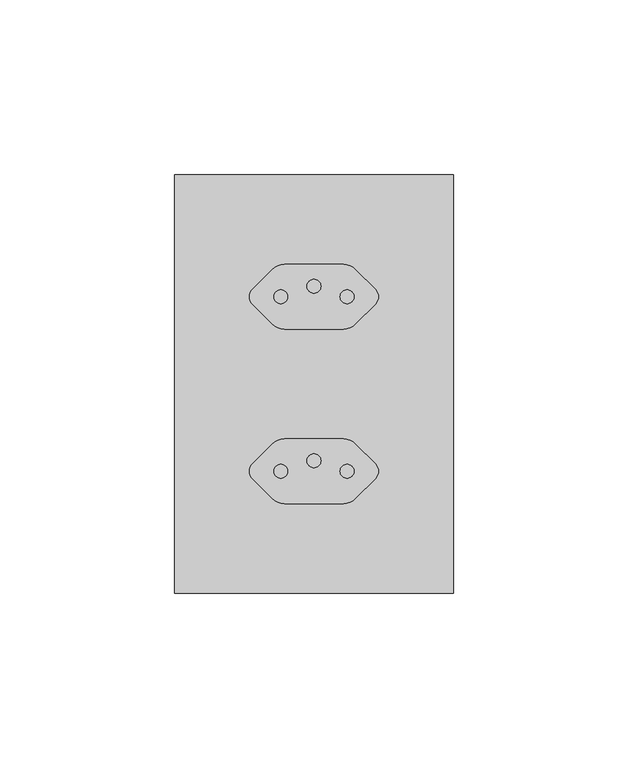
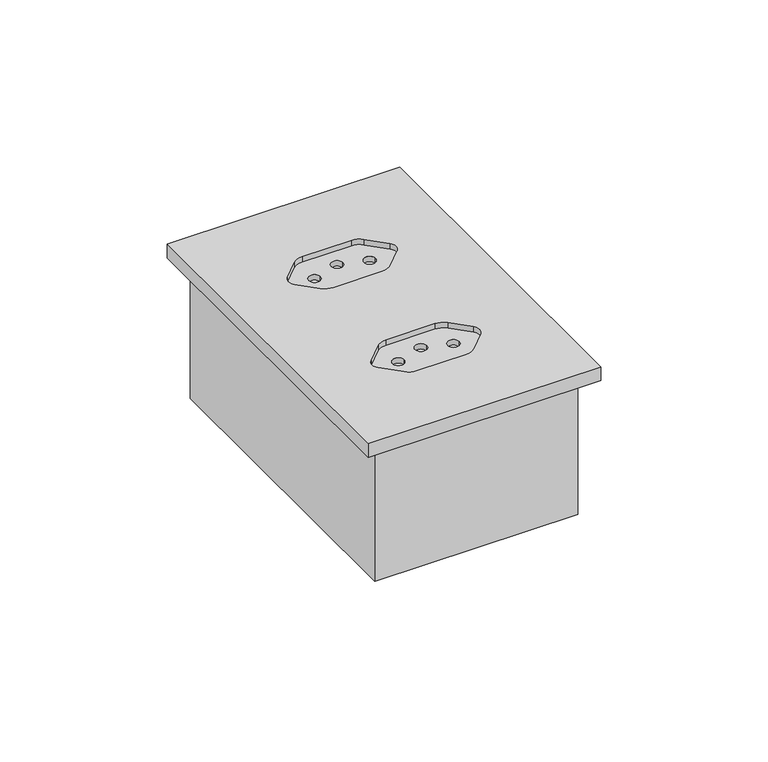
"""IFC4 building model written with IfcOpenShell, lengths in millimetres: proxy geometry, CAIXA VERTICE V7 : Tomada 10A 2s."""

from ifc_helpers import new_model, si_unit, frame, origin, place, context, project, spatial, polyline, circle_curve, faceted_brep, source, transform, mapped, element, save
from ifc_brep_helpers import plane_surface, revolved_surface, advanced_brep


def electrical_fixtures_e68da447(model_context):
    return source(origin(), model_context, "Body", "SolidModel", [
        faceted_brep([(33.0, 1047.0, -48.0), (33.0, 1153.0, -48.0), (-33.0, 1153.0, -48.0), (-33.0, 1047.0, -48.0), (35.0, 1155.0, -50.0), (35.0, 1045.0, -50.0), (-35.0, 1045.0, -50.0), (-35.0, 1155.0, -50.0), (-35.0, 1155.0, 0.0), (35.0, 1155.0, 0.0), (-35.0, 1045.0, 0.0), (35.0, 1045.0, 0.0), (33.0, 1153.0, 0.0), (33.0, 1047.0, 0.0), (-33.0, 1047.0, 0.0), (-33.0, 1153.0, 0.0)], [[[0, 1, 2, 3]], [[4, 5, 6, 7]], [[4, 7, 8, 9]], [[8, 7, 6, 10]], [[10, 6, 5, 11]], [[11, 5, 4, 9]], [[9, 8, 10, 11], [12, 13, 14, 15]], [[13, 12, 1, 0]], [[14, 13, 0, 3]], [[15, 14, 3, 2]], [[12, 15, 2, 1]]]),
        advanced_brep(
        [(40.0, 1160.0, 5.0), (-40.0, 1160.0, 5.0), (-40.0, 1040.0, 5.0), (40.0, 1040.0, 5.0), (8.4215729, 1115.75, 5.0), (-8.4215729, 1115.75, 5.0), (-11.9571068, 1117.2144661, 5.0), (-17.6213203, 1122.8786797, 5.0), (-17.6213203, 1127.1213203, 5.0), (-11.9571068, 1132.7855339, 5.0), (-8.4215729, 1134.25, 5.0), (8.4215729, 1134.25, 5.0), (11.9571068, 1132.7855339, 5.0), (17.6213203, 1127.1213203, 5.0), (17.6213203, 1122.8786797, 5.0), (11.9571068, 1117.2144661, 5.0), (8.4215729, 1065.75, 5.0), (-8.4215729, 1065.75, 5.0), (-11.9571068, 1067.2144661, 5.0), (-17.6213203, 1072.8786797, 5.0), (-17.6213203, 1077.1213203, 5.0), (-11.9571068, 1082.7855339, 5.0), (-8.4215729, 1084.25, 5.0), (8.4215729, 1084.25, 5.0), (11.9571068, 1082.7855339, 5.0), (17.6213203, 1077.1213203, 5.0), (17.6213203, 1072.8786797, 5.0), (11.9571068, 1067.2144661, 5.0), (-40.0, 1160.0, 0.0), (40.0, 1160.0, 0.0), (40.0, 1040.0, 0.0), (-40.0, 1040.0, 0.0), (8.4215729, 1115.75, 3.0), (11.9571068, 1117.2144661, 3.0), (17.6213203, 1122.8786797, 3.0), (17.6213203, 1127.1213203, 3.0), (11.9571068, 1132.7855339, 3.0), (8.4215729, 1134.25, 3.0), (-8.4215729, 1134.25, 3.0), (-11.9571068, 1132.7855339, 3.0), (-17.6213203, 1127.1213203, 3.0), (-17.6213203, 1122.8786797, 3.0), (-11.9571068, 1117.2144661, 3.0), (-8.4215729, 1115.75, 3.0), (-7.5, 1125.0, 3.0), (-11.5, 1125.0, 3.0), (11.5, 1125.0, 3.0), (7.5, 1125.0, 3.0), (2.0, 1128.0, 3.0), (-2.0, 1128.0, 3.0), (-11.5, 1125.0, 1.0), (-7.5, 1125.0, 1.0), (7.5, 1125.0, 1.0), (11.5, 1125.0, 1.0), (-2.0, 1128.0, 1.0), (2.0, 1128.0, 1.0), (8.4215729, 1065.75, 3.0), (11.9571068, 1067.2144661, 3.0), (17.6213203, 1072.8786797, 3.0), (17.6213203, 1077.1213203, 3.0), (11.9571068, 1082.7855339, 3.0), (8.4215729, 1084.25, 3.0), (-8.4215729, 1084.25, 3.0), (-11.9571068, 1082.7855339, 3.0), (-17.6213203, 1077.1213203, 3.0), (-17.6213203, 1072.8786797, 3.0), (-11.9571068, 1067.2144661, 3.0), (-8.4215729, 1065.75, 3.0), (-7.5, 1075.0, 3.0), (-11.5, 1075.0, 3.0), (11.5, 1075.0, 3.0), (7.5, 1075.0, 3.0), (2.0, 1078.0, 3.0), (-2.0, 1078.0, 3.0), (-11.5, 1075.0, 1.0), (-7.5, 1075.0, 1.0), (7.5, 1075.0, 1.0), (11.5, 1075.0, 1.0), (-2.0, 1078.0, 1.0), (2.0, 1078.0, 1.0)],
        [
            (0, 1),
            (1, 2),
            (2, 3),
            (3, 0),
            (4, 5),
            (5, 6, circle_curve(frame((-8.4215729, 1120.75, 5.0), z_axis=(0.0, 0.0, -1.0), x_axis=(-1.0, 0.0, 0.0)), 5.0)),
            (6, 7),
            (7, 8, circle_curve(frame((-15.5, 1125.0, 5.0), z_axis=(0.0, 0.0, -1.0), x_axis=(-1.0, 0.0, 0.0)), 3.0)),
            (8, 9),
            (9, 10, circle_curve(frame((-8.4215729, 1129.25, 5.0), z_axis=(0.0, 0.0, -1.0), x_axis=(-1.0, 0.0, 0.0)), 5.0)),
            (10, 11),
            (11, 12, circle_curve(frame((8.4215729, 1129.25, 5.0), z_axis=(0.0, 0.0, -1.0), x_axis=(-1.0, 0.0, 0.0)), 5.0)),
            (12, 13),
            (13, 14, circle_curve(frame((15.5, 1125.0, 5.0), z_axis=(0.0, 0.0, -1.0), x_axis=(-1.0, 0.0, 0.0)), 3.0)),
            (14, 15),
            (15, 4, circle_curve(frame((8.4215729, 1120.75, 5.0), z_axis=(0.0, 0.0, -1.0), x_axis=(-1.0, 0.0, 0.0)), 5.0)),
            (16, 17),
            (17, 18, circle_curve(frame((-8.4215729, 1070.75, 5.0), z_axis=(0.0, 0.0, -1.0), x_axis=(-1.0, 0.0, 0.0)), 5.0)),
            (18, 19),
            (19, 20, circle_curve(frame((-15.5, 1075.0, 5.0), z_axis=(0.0, 0.0, -1.0), x_axis=(-1.0, 0.0, 0.0)), 3.0)),
            (20, 21),
            (21, 22, circle_curve(frame((-8.4215729, 1079.25, 5.0), z_axis=(0.0, 0.0, -1.0), x_axis=(-1.0, 0.0, 0.0)), 5.0)),
            (22, 23),
            (23, 24, circle_curve(frame((8.4215729, 1079.25, 5.0), z_axis=(0.0, 0.0, -1.0), x_axis=(-1.0, 0.0, 0.0)), 5.0)),
            (24, 25),
            (25, 26, circle_curve(frame((15.5, 1075.0, 5.0), z_axis=(0.0, 0.0, -1.0), x_axis=(-1.0, 0.0, 0.0)), 3.0)),
            (26, 27),
            (27, 16, circle_curve(frame((8.4215729, 1070.75, 5.0), z_axis=(0.0, 0.0, -1.0), x_axis=(-1.0, 0.0, 0.0)), 5.0)),
            (28, 29),
            (29, 30),
            (30, 31),
            (31, 28),
            (0, 29),
            (28, 1),
            (31, 2),
            (30, 3),
            (32, 33, circle_curve(frame((8.4215729, 1120.75, 3.0), z_axis=(0.0, 0.0, 1.0), x_axis=(-1.0, 0.0, 0.0)), 5.0)),
            (33, 34),
            (34, 35, circle_curve(frame((15.5, 1125.0, 3.0), z_axis=(0.0, 0.0, 1.0), x_axis=(-1.0, 0.0, 0.0)), 3.0)),
            (35, 36),
            (36, 37, circle_curve(frame((8.4215729, 1129.25, 3.0), z_axis=(0.0, 0.0, 1.0), x_axis=(-1.0, 0.0, 0.0)), 5.0)),
            (37, 38),
            (38, 39, circle_curve(frame((-8.4215729, 1129.25, 3.0), z_axis=(0.0, 0.0, 1.0), x_axis=(-1.0, 0.0, 0.0)), 5.0)),
            (39, 40),
            (40, 41, circle_curve(frame((-15.5, 1125.0, 3.0), z_axis=(0.0, 0.0, 1.0), x_axis=(-1.0, 0.0, 0.0)), 3.0)),
            (41, 42),
            (42, 43, circle_curve(frame((-8.4215729, 1120.75, 3.0), z_axis=(0.0, 0.0, 1.0), x_axis=(-1.0, 0.0, 0.0)), 5.0)),
            (43, 32),
            (44, 45, circle_curve(frame((-9.5, 1125.0, 3.0), z_axis=(0.0, 0.0, -1.0), x_axis=(1.0, 2.301812013077709e-12, 0.0)), 2.0)),
            (45, 44, circle_curve(frame((-9.5, 1125.0, 3.0), z_axis=(0.0, 0.0, -1.0), x_axis=(1.0, 2.301812013077709e-12, 0.0)), 2.0)),
            (46, 47, circle_curve(frame((9.5, 1125.0, 3.0), z_axis=(0.0, 0.0, -1.0), x_axis=(1.0, 2.301812013077709e-12, 0.0)), 2.0)),
            (47, 46, circle_curve(frame((9.5, 1125.0, 3.0), z_axis=(0.0, 0.0, -1.0), x_axis=(1.0, 2.301812013077709e-12, 0.0)), 2.0)),
            (48, 49, circle_curve(frame((0.0, 1128.0, 3.0), z_axis=(0.0, 0.0, -1.0), x_axis=(1.0, 2.301812013077709e-12, 0.0)), 2.0)),
            (49, 48, circle_curve(frame((0.0, 1128.0, 3.0), z_axis=(0.0, 0.0, -1.0), x_axis=(1.0, 2.301812013077709e-12, 0.0)), 2.0)),
            (43, 5),
            (4, 32),
            (42, 6),
            (41, 7),
            (40, 8),
            (39, 9),
            (38, 10),
            (37, 11),
            (36, 12),
            (35, 13),
            (34, 14),
            (33, 15),
            (50, 51, circle_curve(frame((-9.5, 1125.0, 1.0), z_axis=(0.0, 0.0, 1.0), x_axis=(1.0, 2.301812013077709e-12, 0.0)), 2.0)),
            (51, 50, circle_curve(frame((-9.5, 1125.0, 1.0), z_axis=(0.0, 0.0, 1.0), x_axis=(1.0, 2.301812013077709e-12, 0.0)), 2.0)),
            (52, 53, circle_curve(frame((9.5, 1125.0, 1.0), z_axis=(0.0, 0.0, 1.0), x_axis=(1.0, 2.301812013077709e-12, 0.0)), 2.0)),
            (53, 52, circle_curve(frame((9.5, 1125.0, 1.0), z_axis=(0.0, 0.0, 1.0), x_axis=(1.0, 2.301812013077709e-12, 0.0)), 2.0)),
            (54, 55, circle_curve(frame((0.0, 1128.0, 1.0), z_axis=(0.0, 0.0, 1.0), x_axis=(1.0, 2.301812013077709e-12, 0.0)), 2.0)),
            (55, 54, circle_curve(frame((0.0, 1128.0, 1.0), z_axis=(0.0, 0.0, 1.0), x_axis=(1.0, 2.301812013077709e-12, 0.0)), 2.0)),
            (44, 51),
            (50, 45),
            (46, 53),
            (52, 47),
            (48, 55),
            (54, 49),
            (56, 57, circle_curve(frame((8.4215729, 1070.75, 3.0), z_axis=(0.0, 0.0, 1.0), x_axis=(-1.0, 0.0, 0.0)), 5.0)),
            (57, 58),
            (58, 59, circle_curve(frame((15.5, 1075.0, 3.0), z_axis=(0.0, 0.0, 1.0), x_axis=(-1.0, 0.0, 0.0)), 3.0)),
            (59, 60),
            (60, 61, circle_curve(frame((8.4215729, 1079.25, 3.0), z_axis=(0.0, 0.0, 1.0), x_axis=(-1.0, 0.0, 0.0)), 5.0)),
            (61, 62),
            (62, 63, circle_curve(frame((-8.4215729, 1079.25, 3.0), z_axis=(0.0, 0.0, 1.0), x_axis=(-1.0, 0.0, 0.0)), 5.0)),
            (63, 64),
            (64, 65, circle_curve(frame((-15.5, 1075.0, 3.0), z_axis=(0.0, 0.0, 1.0), x_axis=(-1.0, 0.0, 0.0)), 3.0)),
            (65, 66),
            (66, 67, circle_curve(frame((-8.4215729, 1070.75, 3.0), z_axis=(0.0, 0.0, 1.0), x_axis=(-1.0, 0.0, 0.0)), 5.0)),
            (67, 56),
            (68, 69, circle_curve(frame((-9.5, 1075.0, 3.0), z_axis=(0.0, 0.0, -1.0), x_axis=(1.0, 2.301812013077709e-12, 0.0)), 2.0)),
            (69, 68, circle_curve(frame((-9.5, 1075.0, 3.0), z_axis=(0.0, 0.0, -1.0), x_axis=(1.0, 2.301812013077709e-12, 0.0)), 2.0)),
            (70, 71, circle_curve(frame((9.5, 1075.0, 3.0), z_axis=(0.0, 0.0, -1.0), x_axis=(1.0, 2.301812013077709e-12, 0.0)), 2.0)),
            (71, 70, circle_curve(frame((9.5, 1075.0, 3.0), z_axis=(0.0, 0.0, -1.0), x_axis=(1.0, 2.301812013077709e-12, 0.0)), 2.0)),
            (72, 73, circle_curve(frame((0.0, 1078.0, 3.0), z_axis=(0.0, 0.0, -1.0), x_axis=(1.0, 2.301812013077709e-12, 0.0)), 2.0)),
            (73, 72, circle_curve(frame((0.0, 1078.0, 3.0), z_axis=(0.0, 0.0, -1.0), x_axis=(1.0, 2.301812013077709e-12, 0.0)), 2.0)),
            (67, 17),
            (16, 56),
            (66, 18),
            (65, 19),
            (64, 20),
            (63, 21),
            (62, 22),
            (61, 23),
            (60, 24),
            (59, 25),
            (58, 26),
            (57, 27),
            (74, 75, circle_curve(frame((-9.5, 1075.0, 1.0), z_axis=(0.0, 0.0, 1.0), x_axis=(1.0, 2.301812013077709e-12, 0.0)), 2.0)),
            (75, 74, circle_curve(frame((-9.5, 1075.0, 1.0), z_axis=(0.0, 0.0, 1.0), x_axis=(1.0, 2.301812013077709e-12, 0.0)), 2.0)),
            (76, 77, circle_curve(frame((9.5, 1075.0, 1.0), z_axis=(0.0, 0.0, 1.0), x_axis=(1.0, 2.301812013077709e-12, 0.0)), 2.0)),
            (77, 76, circle_curve(frame((9.5, 1075.0, 1.0), z_axis=(0.0, 0.0, 1.0), x_axis=(1.0, 2.301812013077709e-12, 0.0)), 2.0)),
            (78, 79, circle_curve(frame((0.0, 1078.0, 1.0), z_axis=(0.0, 0.0, 1.0), x_axis=(1.0, 2.301812013077709e-12, 0.0)), 2.0)),
            (79, 78, circle_curve(frame((0.0, 1078.0, 1.0), z_axis=(0.0, 0.0, 1.0), x_axis=(1.0, 2.301812013077709e-12, 0.0)), 2.0)),
            (68, 75),
            (74, 69),
            (70, 77),
            (76, 71),
            (72, 79),
            (78, 73),
        ],
        [
            plane_surface(frame((-60.0, 1160.0, 5.0), z_axis=(0.0, 0.0, 1.0), x_axis=(-1.0, 0.0, 0.0))),
            plane_surface(frame((-60.0, 1160.0, 0.0), z_axis=(0.0, 0.0, -1.0), x_axis=(1.0, 0.0, 0.0))),
            plane_surface(frame((40.0, 1160.0, 5.0), z_axis=(0.0, 1.0, 0.0), x_axis=(0.0, 0.0, -1.0))),
            plane_surface(frame((-40.0, 1160.0, 5.0), z_axis=(-1.0, 0.0, 0.0), x_axis=(0.0, 0.0, -1.0))),
            plane_surface(frame((-40.0, 1040.0, 5.0), z_axis=(0.0, -1.0, 0.0), x_axis=(0.0, 0.0, -1.0))),
            plane_surface(frame((40.0, 1040.0, 5.0), z_axis=(1.0, 0.0, 0.0), x_axis=(0.0, 0.0, -1.0))),
            plane_surface(frame((3.4215729, 1120.75, 3.0), z_axis=(0.0, 0.0, 1.0), x_axis=(0.0, 1.0, 0.0))),
            plane_surface(frame((-8.4215729, 1115.75, 5.0), z_axis=(0.0, 1.0, 0.0), x_axis=(0.0, 0.0, -1.0))),
            revolved_surface(polyline([(-13.4215729, 1120.75, 5.0), (-13.4215729, 1120.75, 3.0)]), (-8.4215729, 1120.75, 3.0), (0.0, 0.0, 1.0)),
            plane_surface(frame((-17.6213203, 1122.8786797, 5.0), z_axis=(0.7071067811865045, 0.7071067811865905, 0.0), x_axis=(0.0, 0.0, -1.0))),
            revolved_surface(polyline([(-18.5, 1125.0, 5.0), (-18.5, 1125.0, 3.0)]), (-15.5, 1125.0, 3.0), (0.0, 0.0, 1.0)),
            plane_surface(frame((-11.9571068, 1132.7855339, 5.0), z_axis=(0.7071067811865515, -0.7071067811865437, 0.0), x_axis=(0.0, 0.0, -1.0))),
            revolved_surface(polyline([(-13.4215729, 1129.25, 5.0), (-13.4215729, 1129.25, 3.0)]), (-8.4215729, 1129.25, 3.0), (0.0, 0.0, 1.0)),
            plane_surface(frame((8.4215729, 1134.25, 5.0), z_axis=(0.0, -1.0, 0.0), x_axis=(0.0, 0.0, -1.0))),
            revolved_surface(polyline([(3.4215728999999993, 1129.25, 5.0), (3.4215728999999993, 1129.25, 3.0)]), (8.4215729, 1129.25, 3.0), (0.0, 0.0, 1.0)),
            plane_surface(frame((17.6213203, 1127.1213203, 5.0), z_axis=(-0.7071067811865307, -0.7071067811865643, 0.0), x_axis=(0.0, 0.0, -1.0))),
            revolved_surface(polyline([(12.5, 1125.0, 5.0), (12.5, 1125.0, 3.0)]), (15.5, 1125.0, 3.0), (0.0, 0.0, 1.0)),
            plane_surface(frame((11.9571068, 1117.2144661, 5.0), z_axis=(-0.7071067811865893, 0.7071067811865058, 0.0), x_axis=(0.0, 0.0, -1.0))),
            revolved_surface(polyline([(3.4215728999999993, 1120.75, 5.0), (3.4215728999999993, 1120.75, 3.0)]), (8.4215729, 1120.75, 3.0), (0.0, 0.0, 1.0)),
            plane_surface(frame((-7.5, 1125.0, 1.0), z_axis=(0.0, 0.0, 1.0), x_axis=(2.301812013077709e-12, -1.0, 0.0))),
            revolved_surface(polyline([(-7.5, 1125.0000000000045, 3.0), (-7.5, 1125.0000000000045, 1.0)]), (-9.5, 1125.0, 1.0), (0.0, 0.0, 1.0)),
            revolved_surface(polyline([(11.5, 1125.0000000000045, 3.0), (11.5, 1125.0000000000045, 1.0)]), (9.5, 1125.0, 5.0), (0.0, 0.0, 1.0)),
            revolved_surface(polyline([(2.0, 1128.0000000000045, 3.0), (2.0, 1128.0000000000045, 1.0)]), (0.0, 1128.0, 5.0), (0.0, 0.0, 1.0)),
            plane_surface(frame((3.4215729, 1070.75, 3.0), z_axis=(0.0, 0.0, 1.0), x_axis=(0.0, 1.0, 0.0))),
            plane_surface(frame((-8.4215729, 1065.75, 5.0), z_axis=(0.0, 1.0, 0.0), x_axis=(0.0, 0.0, -1.0))),
            revolved_surface(polyline([(-13.4215729, 1070.75, 5.0), (-13.4215729, 1070.75, 3.0)]), (-8.4215729, 1070.75, 3.0), (0.0, 0.0, 1.0)),
            plane_surface(frame((-17.6213203, 1072.8786797, 5.0), z_axis=(0.7071067811865045, 0.7071067811865905, 0.0), x_axis=(0.0, 0.0, -1.0))),
            revolved_surface(polyline([(-18.5, 1075.0, 5.0), (-18.5, 1075.0, 3.0)]), (-15.5, 1075.0, 3.0), (0.0, 0.0, 1.0)),
            plane_surface(frame((-11.9571068, 1082.7855339, 5.0), z_axis=(0.7071067811865515, -0.7071067811865437, 0.0), x_axis=(0.0, 0.0, -1.0))),
            revolved_surface(polyline([(-13.4215729, 1079.25, 5.0), (-13.4215729, 1079.25, 3.0)]), (-8.4215729, 1079.25, 3.0), (0.0, 0.0, 1.0)),
            plane_surface(frame((8.4215729, 1084.25, 5.0), z_axis=(0.0, -1.0, 0.0), x_axis=(0.0, 0.0, -1.0))),
            revolved_surface(polyline([(3.4215728999999993, 1079.25, 5.0), (3.4215728999999993, 1079.25, 3.0)]), (8.4215729, 1079.25, 3.0), (0.0, 0.0, 1.0)),
            plane_surface(frame((17.6213203, 1077.1213203, 5.0), z_axis=(-0.7071067811865307, -0.7071067811865643, 0.0), x_axis=(0.0, 0.0, -1.0))),
            revolved_surface(polyline([(12.5, 1075.0, 5.0), (12.5, 1075.0, 3.0)]), (15.5, 1075.0, 3.0), (0.0, 0.0, 1.0)),
            plane_surface(frame((11.9571068, 1067.2144661, 5.0), z_axis=(-0.7071067811865893, 0.7071067811865058, 0.0), x_axis=(0.0, 0.0, -1.0))),
            revolved_surface(polyline([(3.4215728999999993, 1070.75, 5.0), (3.4215728999999993, 1070.75, 3.0)]), (8.4215729, 1070.75, 3.0), (0.0, 0.0, 1.0)),
            plane_surface(frame((-7.5, 1075.0, 1.0), z_axis=(0.0, 0.0, 1.0), x_axis=(2.301812013077709e-12, -1.0, 0.0))),
            revolved_surface(polyline([(-7.5, 1075.0000000000045, 3.0), (-7.5, 1075.0000000000045, 1.0)]), (-9.5, 1075.0, 1.0), (0.0, 0.0, 1.0)),
            revolved_surface(polyline([(11.5, 1075.0000000000045, 3.0), (11.5, 1075.0000000000045, 1.0)]), (9.5, 1075.0, 5.0), (0.0, 0.0, 1.0)),
            revolved_surface(polyline([(2.0, 1078.0000000000045, 3.0), (2.0, 1078.0000000000045, 1.0)]), (0.0, 1078.0, 5.0), (0.0, 0.0, 1.0)),
        ],
        [
            (0, [[1, 2, 3, 4], [5, 6, 7, 8, 9, 10, 11, 12, 13, 14, 15, 16], [17, 18, 19, 20, 21, 22, 23, 24, 25, 26, 27, 28]]),
            (1, [[29, 30, 31, 32]]),
            (2, [[-1, 33, -29, 34]]),
            (3, [[-2, -34, -32, 35]]),
            (4, [[-3, -35, -31, 36]]),
            (5, [[-4, -36, -30, -33]]),
            (6, [[37, 38, 39, 40, 41, 42, 43, 44, 45, 46, 47, 48], [49, 50], [51, 52], [53, 54]]),
            (7, [[-48, 55, -5, 56]]),
            (8, [[-47, 57, -6, -55]]),
            (9, [[-46, 58, -7, -57]]),
            (10, [[-45, 59, -8, -58]]),
            (11, [[-44, 60, -9, -59]]),
            (12, [[-43, 61, -10, -60]]),
            (13, [[-42, 62, -11, -61]]),
            (14, [[-41, 63, -12, -62]]),
            (15, [[-40, 64, -13, -63]]),
            (16, [[-39, 65, -14, -64]]),
            (17, [[-38, 66, -15, -65]]),
            (18, [[-37, -56, -16, -66]]),
            (19, [[67, 68]]),
            (19, [[69, 70]]),
            (19, [[71, 72]]),
            (20, [[-49, 73, -67, 74]]),
            (20, [[-50, -74, -68, -73]]),
            (21, [[-51, 75, -69, 76]]),
            (21, [[-52, -76, -70, -75]]),
            (22, [[-53, 77, -71, 78]]),
            (22, [[-54, -78, -72, -77]]),
            (23, [[79, 80, 81, 82, 83, 84, 85, 86, 87, 88, 89, 90], [91, 92], [93, 94], [95, 96]]),
            (24, [[-90, 97, -17, 98]]),
            (25, [[-89, 99, -18, -97]]),
            (26, [[-88, 100, -19, -99]]),
            (27, [[-87, 101, -20, -100]]),
            (28, [[-86, 102, -21, -101]]),
            (29, [[-85, 103, -22, -102]]),
            (30, [[-84, 104, -23, -103]]),
            (31, [[-83, 105, -24, -104]]),
            (32, [[-82, 106, -25, -105]]),
            (33, [[-81, 107, -26, -106]]),
            (34, [[-80, 108, -27, -107]]),
            (35, [[-79, -98, -28, -108]]),
            (36, [[109, 110]]),
            (36, [[111, 112]]),
            (36, [[113, 114]]),
            (37, [[-91, 115, -109, 116]]),
            (37, [[-92, -116, -110, -115]]),
            (38, [[-93, 117, -111, 118]]),
            (38, [[-94, -118, -112, -117]]),
            (39, [[-95, 119, -113, 120]]),
            (39, [[-96, -120, -114, -119]]),
        ],
    ),
    ])


if __name__ == "__main__":
    model = new_model("IFC4")
    model_context = context("Model", 3, world=origin())
    ifc_project = project(units=[si_unit("LENGTHUNIT", "METRE", prefix="MILLI")], contexts=[model_context])
    site = spatial("IfcSite", under=ifc_project)
    building = spatial("IfcBuilding", under=site)
    placement = place(None, origin())
    electrical_fixtures_shape = electrical_fixtures_e68da447(model_context)
    element("IfcBuildingElementProxy", 1, Name="CAIXA VERTICE V7 : Tomada 10A 2s", ObjectType="CAIXA VERTICE V7 : Tomada 10A 2s", at=placement, inside=building, context=model_context, shape_type="MappedRepresentation", body=[
        mapped(electrical_fixtures_shape, transform((0.0, 0.0, 0.0), x_axis=(1.0, 0.0, 0.0), y_axis=(0.0, 1.0, 0.0), z_axis=(0.0, 0.0, 1.0))),
    ])
    save(model, "model.ifc")

# Revit data of these elements
# Type "CAIXA VERTICE V7 : Tomada 10A 2s"
#   URL = "www.facebook.com/verticetreinamentos"
#   SEÇÃO [instance default] = ""
#   Rotação [instance default] = 0.00°
#   LARGURA DA TAMPA = 0.08 m
#   BORDA = 0.01 m
#   ALTURA DE INSTALAÇÃO [instance default] = 1.10 m
#   Distância Anotação [instance default] = 0.0015 m
#   ALTURA DA TAMPA = 0.12 m
#   Vertical [instance default] = yes
#   VER SEÇÃO [instance default] = no
#   SHADE ESQ [instance default] = no
#   SHADE DIR [instance default] = yes
#   HORIZONTAL [instance default] = no
#   ANDAR COM A LEGENDA [instance default] = 0
#   Material Tampa [instance default] = Plástico, branco opaco
#   Caixa = element 1798515
#   Anotação = element 1798529
#   Default Elevation = 0
# Element 1 (IfcBuildingElementProxy, "CAIXA VERTICE V7 : Tomada 10A 2s")
#   Materials on its faces: "Plástico, branco opaco"
# Materials
#   "Plástico, branco opaco": class "Plástico", colour RGB 120 120 120, transparency 0, Description = "Plastic, generic, opaque white", Cost = 0
